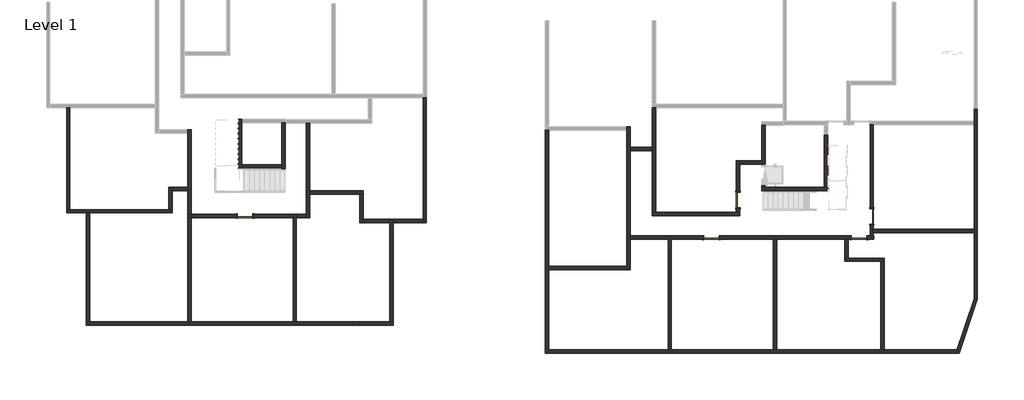
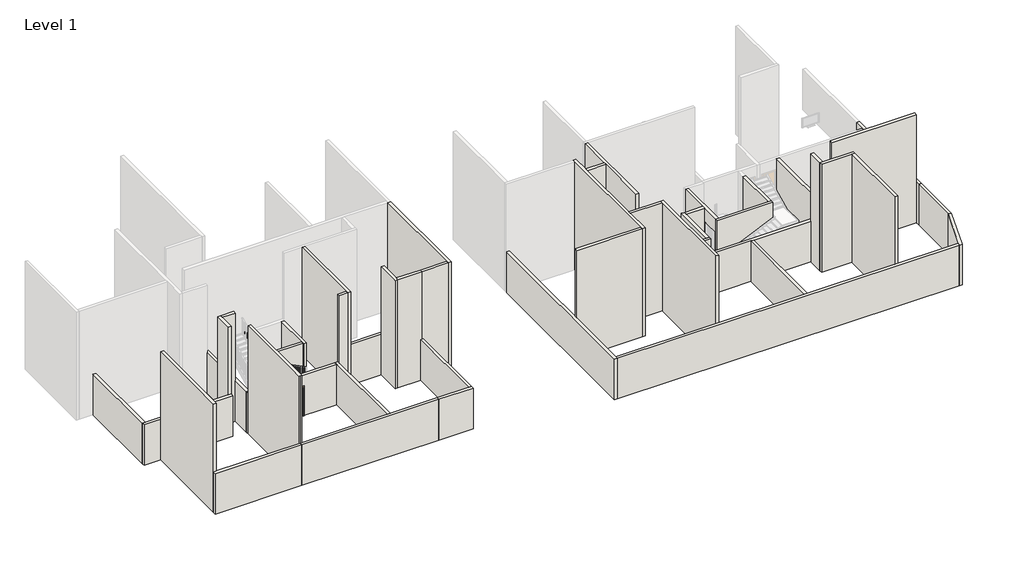
# One storey, part 1 of 3: 47 walls, 5 doors.
"""IFC4 building model written with IfcOpenShell, lengths in millimetres."""

import ifcopenshell
import ifcopenshell.guid

model = None  # the IFC model being written
_history = None  # IfcOwnerHistory: only IFC2X3 demands one
_inside = {}  # id of a spatial element -> (the spatial element, [elements in it])
_under = {}  # id of a project, library or spatial element -> (it, [spatial elements below it])
_declared = {}  # id of a project -> (the project, [libraries it declares])
_typed = {}  # id of a type object -> (the type object, [elements of that type])
_made_of = {}  # id of a material, layer set ... -> (it, [elements and type objects made of it])


def new_model(schema):
    """Start an empty IFC model of exactly this schema.

    Asked for "IFC4X3", IfcOpenShell would pick the latest addendum, in which some entities
    have other attributes; the version numbers below select the first issue.
    IFC2X3 requires an IfcOwnerHistory on every rooted entity: one is made here for all.
    """
    global model, _history
    if schema == "IFC4X3":
        model = ifcopenshell.file(schema_version=(4, 3, 0, 0))
    else:
        model = ifcopenshell.file(schema=schema)
    _inside.clear()
    _under.clear()
    _declared.clear()
    _typed.clear()
    _made_of.clear()
    _history = None
    if model.schema == "IFC2X3":
        org = make("IfcOrganization", Name="unknown")
        user = make(
            "IfcPersonAndOrganization",
            ThePerson=make("IfcPerson", FamilyName="unknown"),
            TheOrganization=org,
        )
        app = make(
            "IfcApplication",
            ApplicationDeveloper=org,
            Version="unknown",
            ApplicationFullName="unknown",
            ApplicationIdentifier="unknown",
        )
        _history = make(
            "IfcOwnerHistory",
            OwningUser=user,
            OwningApplication=app,
            ChangeAction="ADDED",
            CreationDate=0,
        )
    return model


def make(cls, **values):
    """One entity of the class cls with the attributes given. An attribute that is None is left unset."""
    return model.create_entity(
        cls, **{name: value for name, value in values.items() if value is not None}
    )


def rooted(cls, **values):
    """An entity with a GlobalId (a new one), such as an element, a storey or a relation."""
    return make(cls, GlobalId=ifcopenshell.guid.new(), OwnerHistory=_history, **values)


def si_unit(unit_type, name, prefix=None):
    """IfcSIUnit, for example si_unit("LENGTHUNIT", "METRE", prefix="MILLI")."""
    return make("IfcSIUnit", UnitType=unit_type, Prefix=prefix, Name=name)


def assignment(units):
    """IfcUnitAssignment: the units of a project."""
    return None if units is None else make("IfcUnitAssignment", Units=units)


def point(xyz):
    """IfcCartesianPoint."""
    return None if xyz is None else make("IfcCartesianPoint", Coordinates=xyz)


def direction(xyz):
    """IfcDirection."""
    return None if xyz is None else make("IfcDirection", DirectionRatios=xyz)


def frame(location, z_axis=None, x_axis=None):
    """IfcAxis2Placement3D, a coordinate frame: its origin and axes. An axis left out is left unset."""
    return make(
        "IfcAxis2Placement3D",
        Location=point(location),
        Axis=direction(z_axis),
        RefDirection=direction(x_axis),
    )


def origin():
    """The frame at (0, 0, 0) with its axes left unset."""
    return frame((0.0, 0.0, 0.0))


def origin_with_axes():
    """The frame at (0, 0, 0) with the z axis (0, 0, 1) and the x axis (1, 0, 0) written out."""
    return frame((0.0, 0.0, 0.0), z_axis=(0.0, 0.0, 1.0), x_axis=(1.0, 0.0, 0.0))


def place(relative_to, where):
    """IfcLocalPlacement: puts the frame where relative to a parent placement (None: the world)."""
    return make(
        "IfcLocalPlacement", PlacementRelTo=relative_to, RelativePlacement=where
    )


def context(
    kind, dimensions, precision=None, world=None, true_north=None, identifier=None
):
    """IfcGeometricRepresentationContext, for example the 3D "Model" context."""
    return make(
        "IfcGeometricRepresentationContext",
        ContextIdentifier=identifier,
        ContextType=kind,
        CoordinateSpaceDimension=dimensions,
        Precision=precision,
        WorldCoordinateSystem=world,
        TrueNorth=true_north,
    )


def project(units=None, contexts=None):
    """IfcProject with its units and contexts."""
    return rooted(
        "IfcProject",
        Name="project",
        RepresentationContexts=contexts,
        UnitsInContext=assignment(units),
    )


def spatial(cls, under=None, at=None, **own):
    """A site, building, storey or space (cls), placed at a placement, below another one or the project."""
    s = rooted(cls, ObjectPlacement=at, **own)
    if under is not None:
        _under.setdefault(under.id(), (under, []))[1].append(s)
    return s


def polyline(points):
    """IfcPolyline through the points."""
    return make("IfcPolyline", Points=[point(p) for p in points])


def outline(outer, holes=None, kind="AREA"):
    """IfcArbitraryClosedProfileDef: a profile drawn as a closed curve; with holes, ...WithVoids."""
    if holes is None:
        return make("IfcArbitraryClosedProfileDef", ProfileType=kind, OuterCurve=outer)
    return make(
        "IfcArbitraryProfileDefWithVoids",
        ProfileType=kind,
        OuterCurve=outer,
        InnerCurves=holes,
    )


def extrude(swept, where, along, depth):
    """IfcExtrudedAreaSolid: the profile swept, set in the frame where, extruded along a direction by depth."""
    return make(
        "IfcExtrudedAreaSolid",
        SweptArea=swept,
        Position=where,
        ExtrudedDirection=direction(along),
        Depth=depth,
    )


def faces_of(points, faces, orient=None, outer=None):
    """IfcFace entities. A face is a list of loops; a loop is a list of indices into points, from 0.

    orient and outer hold one flag for each loop. By default every Orientation is true, the
    first loop of a face is its IfcFaceOuterBound and the others are IfcFaceBound.
    """
    made = []
    for i, loops in enumerate(faces):
        bounds = []
        for j, loop in enumerate(loops):
            is_outer = j == 0 if outer is None else outer[i][j]
            bounds.append(
                make(
                    "IfcFaceOuterBound" if is_outer else "IfcFaceBound",
                    Bound=make("IfcPolyLoop", Polygon=[points[k] for k in loop]),
                    Orientation=True if orient is None else orient[i][j],
                )
            )
        made.append(make("IfcFace", Bounds=bounds))
    return made


def faceted_brep(points, faces, orient=None, outer=None, voids=None):
    """IfcFacetedBrep: a solid bounded by flat faces; with voids (closed shells), ...WithVoids."""
    shared = [point(p) for p in points]
    hull = make("IfcClosedShell", CfsFaces=faces_of(shared, faces, orient, outer))
    if voids is None:
        return make("IfcFacetedBrep", Outer=hull)
    return make(
        "IfcFacetedBrepWithVoids",
        Outer=hull,
        Voids=[
            make(cls, CfsFaces=faces_of(shared, fs, o, b)) for cls, fs, o, b in voids
        ],
    )


def shape(context_of_items, identifier, shape_type, items):
    """IfcShapeRepresentation: the items that make up one representation, for example the "Body"."""
    return make(
        "IfcShapeRepresentation",
        ContextOfItems=context_of_items,
        RepresentationIdentifier=identifier,
        RepresentationType=shape_type,
        Items=items,
    )


def source(mapping_origin, context_of_items, identifier, shape_type, items):
    """IfcRepresentationMap: a shape defined once, which mapped items show again and again."""
    return make(
        "IfcRepresentationMap",
        MappingOrigin=mapping_origin,
        MappedRepresentation=shape(context_of_items, identifier, shape_type, items),
    )


def transform(
    local_origin,
    x_axis=None,
    y_axis=None,
    z_axis=None,
    scale=None,
    scale2=None,
    scale3=None,
    uniform=True,
):
    """IfcCartesianTransformationOperator3D, or its non-uniform kind. x_axis, y_axis, z_axis: its Axis1, 2, 3."""
    if uniform:
        return make(
            "IfcCartesianTransformationOperator3D",
            Axis1=direction(x_axis),
            Axis2=direction(y_axis),
            LocalOrigin=point(local_origin),
            Scale=scale,
            Axis3=direction(z_axis),
        )
    return make(
        "IfcCartesianTransformationOperator3DnonUniform",
        Axis1=direction(x_axis),
        Axis2=direction(y_axis),
        LocalOrigin=point(local_origin),
        Scale=scale,
        Axis3=direction(z_axis),
        Scale2=scale2,
        Scale3=scale3,
    )


def mapped(mapping_source, mapping_target):
    """IfcMappedItem: shows the shape of a source again, moved by a transform."""
    return make(
        "IfcMappedItem", MappingSource=mapping_source, MappingTarget=mapping_target
    )


def made_of(thing, what):
    """Note that an element or type object is made of a material, layer set ...; save() writes the relation."""
    if what is not None:
        _made_of.setdefault(what.id(), (what, []))[1].append(thing)
    return thing


def element(
    cls,
    number,
    at=None,
    inside=None,
    cuts=None,
    type_object=None,
    material=None,
    context=None,
    identifier="Body",
    shape_type=None,
    held_by="IfcProductDefinitionShape",
    body=None,
    shapes=None,
    **own,
):
    """One element of the class cls, such as IfcWall. Its Tag is "e" and its number.

    at: its placement. inside: the storey or other place that contains it. cuts: it is an
    opening in that element (IfcRelVoidsElement). A single representation is given by context,
    identifier, shape_type and body (its items); several are given by shapes. held_by: the class
    of the entity that holds the representations. save() writes the other relations.
    """
    e = rooted(cls, Tag="e%d" % number, ObjectPlacement=at, **own)
    if body is not None:
        shapes = [shape(context, identifier, shape_type, body)]
    if shapes is not None:
        e.Representation = make(held_by, Representations=shapes)
    if inside is not None:
        _inside.setdefault(inside.id(), (inside, []))[1].append(e)
    if cuts is not None:
        rooted(
            "IfcRelVoidsElement", RelatingBuildingElement=cuts, RelatedOpeningElement=e
        )
    if type_object is not None:
        _typed.setdefault(type_object.id(), (type_object, []))[1].append(e)
    return made_of(e, material)


def aggregate(whole, parts):
    """IfcRelAggregates: a whole, such as a stair, and the parts it consists of."""
    return rooted("IfcRelAggregates", RelatingObject=whole, RelatedObjects=parts)


def save(model, path):
    """Write the relations noted so far, then the file.

    IfcRelAggregates (storeys below a building ...), IfcRelContainedInSpatialStructure (elements
    in a storey), IfcRelDefinesByType, IfcRelAssociatesMaterial and IfcRelDeclares: one each for
    every whole, place, type object, material and project.
    """
    for whole, parts in _under.values():
        aggregate(whole, parts)
    for where, things in _inside.values():
        rooted(
            "IfcRelContainedInSpatialStructure",
            RelatedElements=things,
            RelatingStructure=where,
        )
    for kind, things in _typed.values():
        rooted("IfcRelDefinesByType", RelatedObjects=things, RelatingType=kind)
    for what, things in _made_of.values():
        rooted("IfcRelAssociatesMaterial", RelatedObjects=things, RelatingMaterial=what)
    for by, libraries in _declared.values():
        rooted("IfcRelDeclares", RelatingContext=by, RelatedDefinitions=libraries)
    model.write(path)


def m_single_flush_0915_x_2134mm_727434cd(model_context):
    return source(origin(), model_context, "Body", "SweptSolid", [
        extrude(outline(polyline([(2210.0, -533.5), (0.0, -533.5), (0.0, -457.5), (2134.0, -457.5), (2134.0, 457.5), (0.0, 457.5), (0.0, 533.5), (2210.0, 533.5), (2210.0, -533.5)])), frame((0.0, -125.0, 0.0), z_axis=(0.0, 1.0, 0.0), x_axis=(0.0, 0.0, 1.0)), (0.0, 0.0, 1.0), 25.0),
        extrude(outline(polyline([(2210.0, 533.5), (2210.0, -533.5), (0.0, -533.5), (0.0, -457.5), (2134.0, -457.5), (2134.0, 457.5), (0.0, 457.5), (0.0, 533.5), (2210.0, 533.5)])), frame((0.0, 100.0, 0.0), z_axis=(0.0, 1.0, 0.0), x_axis=(0.0, 0.0, 1.0)), (0.0, 0.0, 1.0), 25.0),
        extrude(outline(polyline([(457.5, -49.0), (457.5, -100.0), (-457.5, -100.0), (-457.5, -49.0), (457.5, -49.0)])), origin_with_axes(), (0.0, 0.0, 1.0), 2134.0),
    ])


def m_single_flush_0915_x_2134mm_6a9e8738(model_context):
    return source(origin(), model_context, "Body", "SweptSolid", [
        extrude(outline(polyline([(2210.0, -533.5), (0.0, -533.5), (0.0, -457.5), (2134.0, -457.5), (2134.0, 457.5), (0.0, 457.5), (0.0, 533.5), (2210.0, 533.5), (2210.0, -533.5)])), frame((0.0, 100.0, 0.0), z_axis=(0.0, 1.0, 0.0), x_axis=(0.0, 0.0, 1.0)), (0.0, 0.0, 1.0), 25.0),
        extrude(outline(polyline([(2210.0, 533.5), (2210.0, -533.5), (0.0, -533.5), (0.0, -457.5), (2134.0, -457.5), (2134.0, 457.5), (0.0, 457.5), (0.0, 533.5), (2210.0, 533.5)])), frame((0.0, -125.0, 0.0), z_axis=(0.0, 1.0, 0.0), x_axis=(0.0, 0.0, 1.0)), (0.0, 0.0, 1.0), 25.0),
        extrude(outline(polyline([(457.5, 49.0), (-457.5, 49.0), (-457.5, 100.0), (457.5, 100.0), (457.5, 49.0)])), origin_with_axes(), (0.0, 0.0, 1.0), 2134.0),
    ])


model = new_model("IFC4")

# Units and contexts
model_context = context("Model", 3, world=origin())
ifc_project = project(units=[si_unit("LENGTHUNIT", "METRE", prefix="MILLI")], contexts=[model_context])

# Site, building, storey
site = spatial("IfcSite", under=ifc_project)
building = spatial("IfcBuilding", under=site)
storey = spatial("IfcBuildingStorey", under=building, Name="Level 1", Elevation=0.0)

# Doors
placement = place(None, origin())
m_single_flush_0915_x_2134mm_shape = m_single_flush_0915_x_2134mm_727434cd(model_context)
element("IfcDoor", 1, ObjectType="M_Single-Flush : 0915 x 2134mm", at=placement, inside=storey, context=model_context, shape_type="MappedRepresentation", body=[
    mapped(m_single_flush_0915_x_2134mm_shape, transform((16170.6041014, -4023.024372, 0.0), x_axis=(0.0, -1.0, 0.0), y_axis=(1.0, 0.0, 0.0), z_axis=(0.0, 0.0, 1.0))),
])
m_single_flush_0915_x_2134mm_2_shape = m_single_flush_0915_x_2134mm_6a9e8738(model_context)
element("IfcDoor", 2, ObjectType="M_Single-Flush : 0915 x 2134mm", at=placement, inside=storey, context=model_context, shape_type="MappedRepresentation", body=[
    mapped(m_single_flush_0915_x_2134mm_2_shape, transform((14602.336337, -6240.0098119, 0.0), x_axis=(-1.0, 0.0, 0.0), y_axis=(0.0, -1.0, 0.0), z_axis=(0.0, 0.0, 1.0))),
])
element("IfcDoor", 3, ObjectType="M_Single-Flush : 0915 x 2134mm", at=placement, inside=storey, context=model_context, shape_type="MappedRepresentation", body=[
    mapped(m_single_flush_0915_x_2134mm_2_shape, transform((24048.8612349, -4982.5098119, 0.0), x_axis=(0.0, -1.0, 0.0), y_axis=(1.0, 0.0, 0.0), z_axis=(0.0, 0.0, 1.0))),
])
element("IfcDoor", 4, ObjectType="M_Single-Flush : 0915 x 2134mm", at=placement, inside=storey, context=model_context, shape_type="MappedRepresentation", body=[
    mapped(m_single_flush_0915_x_2134mm_2_shape, transform((23308.8612349, -6240.0098119, 0.0), x_axis=(-1.0, 0.0, 0.0), y_axis=(0.0, -1.0, 0.0), z_axis=(0.0, 0.0, 1.0))),
])
element("IfcDoor", 5, ObjectType="M_Single-Flush : 0915 x 2134mm", at=placement, inside=storey, context=model_context, shape_type="MappedRepresentation", body=[
    mapped(m_single_flush_0915_x_2134mm_2_shape, transform((-12832.3304233, -4959.1627129, 0.0), x_axis=(-1.0, 0.0, 0.0), y_axis=(0.0, -1.0, 0.0), z_axis=(0.0, 0.0, 1.0))),
])

# Walls
element("IfcWall", 6, ObjectType="Generic - 200mm", at=placement, inside=storey, context=model_context, shape_type="Brep", body=[
    faceted_brep([(30068.8612349, 1319.475628, 0.0), (30068.8612349, 619.475628, 0.0), (30068.8612349, 419.475628, 0.0), (30068.8612349, -5760.0098119, 0.0), (30068.8612349, -5960.0098119, 0.0), (30068.8612349, -6240.0098119, 0.0), (30068.8612349, -6240.0098119, 3000.0), (30068.8612349, 419.475628, 3000.0), (30068.8612349, 619.475628, 3000.0), (30068.8612349, 1319.475628, 3000.0), (30268.8612349, 1319.475628, 0.0), (30268.8612349, 1319.475628, 3000.0), (30268.8612349, -6240.0098119, 3000.0), (30268.8612349, -6240.0098119, 0.0), (30268.3425199, 1319.475628, 0.0), (30069.3799498, -6240.0098119, 0.0), (30069.3799498, -6240.0098119, 3000.0), (30268.3425199, 1319.475628, 3000.0)], [[[0, 1, 2, 3, 4, 5, 6, 7, 8, 9]], [[10, 11, 12, 13]], [[5, 4, 3, 2, 1, 0, 14, 10, 13, 15]], [[6, 5, 15, 13, 12, 16]], [[9, 8, 7, 6, 16, 12, 11, 17]], [[0, 9, 17, 11, 10, 14]]]),
])
element("IfcWall", 7, ObjectType="Generic - 200mm", at=placement, inside=storey, context=model_context, shape_type="Brep", body=[
    faceted_brep([(30069.3799498, -6240.0098119, 0.0), (30069.3799498, -9831.8731192, 0.0), (30069.3799498, -9831.8731192, 3000.0), (30069.3799498, -6240.0098119, 3000.0), (30269.3799498, -6240.0098119, 0.0), (30269.3799498, -6240.0098119, 3000.0), (30269.3799498, -9864.7113693, 3000.0), (30269.3799498, -9864.7113693, 0.0), (30268.8612349, -6240.0098119, 0.0), (30268.8612349, -6240.0098119, 3000.0)], [[[0, 1, 2, 3]], [[4, 5, 6, 7]], [[1, 0, 8, 4, 7]], [[3, 2, 6, 5, 9]], [[0, 3, 9, 5, 4, 8]], [[2, 1, 7, 6]]]),
])
element("IfcWall", 8, ObjectType="Generic - 200mm", at=placement, inside=storey, context=model_context, shape_type="Brep", body=[
    faceted_brep([(21449.836337, -3276.2808257, 0.0), (21249.836337, -3276.2808257, 0.0), (17770.6041014, -3276.2808257, 0.0), (17570.6041014, -3276.2808257, 0.0), (17570.6041014, -3276.2808257, 3000.0), (17770.6041014, -3276.2808257, 3000.0), (21249.836337, -3276.2808257, 3000.0), (21449.836337, -3276.2808257, 3000.0), (21449.836337, -3476.2808257, 0.0), (21449.836337, -3476.2808257, 3000.0), (17570.6041014, -3476.2808257, 3000.0), (17570.6041014, -3476.2808257, 0.0)], [[[0, 1, 2, 3, 4, 5, 6, 7]], [[8, 9, 10, 11]], [[3, 2, 1, 0, 8, 11]], [[7, 6, 5, 4, 10, 9]], [[0, 7, 9, 8]], [[4, 3, 11, 10]]]),
])
element("IfcWall", 9, ObjectType="Generic - 200mm", at=placement, inside=storey, context=model_context, shape_type="SweptSolid", body=[
    extrude(outline(polyline([(18459.836337, -6340.0098119), (18459.836337, -12836.6907835), (18259.836337, -12836.6907835), (18259.836337, -6340.0098119), (18459.836337, -6340.0098119)])), origin_with_axes(), (0.0, 0.0, 1.0), 3000.0),
])
element("IfcWall", 10, ObjectType="Generic - 200mm", at=placement, inside=storey, context=model_context, shape_type="Brep", body=[
    faceted_brep([(29055.3124022, -12836.6907835, 0.0), (24788.8612349, -12836.6907835, 0.0), (24588.8612349, -12836.6907835, 0.0), (18459.836337, -12836.6907835, 0.0), (18259.836337, -12836.6907835, 0.0), (12259.836337, -12836.6907835, 0.0), (12059.836337, -12836.6907835, 0.0), (5043.716007, -12836.6907835, 0.0), (5043.716007, -12836.6907835, 3000.0), (18259.836337, -12836.6907835, 3000.0), (18459.836337, -12836.6907835, 3000.0), (29055.3124022, -12836.6907835, 3000.0), (28987.8162902, -13036.6907835, 0.0), (28987.8162902, -13036.6907835, 3000.0), (5043.716007, -13036.6907835, 3000.0), (5043.716007, -13036.6907835, 0.0)], [[[0, 1, 2, 3, 4, 5, 6, 7, 8, 9, 10, 11]], [[12, 13, 14, 15]], [[7, 6, 5, 4, 3, 2, 1, 0, 12, 15]], [[11, 10, 9, 8, 14, 13]], [[0, 11, 13, 12]], [[8, 7, 15, 14]]]),
])
element("IfcWall", 11, ObjectType="Generic - 200mm", at=placement, inside=storey, context=model_context, shape_type="Brep", body=[
    faceted_brep([(30069.3799498, -9831.8731192, 0.0), (29055.3124022, -12836.6907835, 0.0), (28987.8162902, -13036.6907835, 0.0), (28987.8162902, -13036.6907835, 3000.0), (29055.3124022, -12836.6907835, 3000.0), (30069.3799498, -9831.8731192, 3000.0), (30269.3799498, -9864.7113693, 0.0), (30269.3799498, -9864.7113693, 3000.0), (29198.8985612, -13036.6907835, 3000.0), (29198.8985612, -13036.6907835, 0.0)], [[[0, 1, 2, 3, 4, 5]], [[6, 7, 8, 9]], [[2, 1, 0, 6, 9]], [[5, 4, 3, 8, 7]], [[0, 5, 7, 6]], [[3, 2, 9, 8]]]),
])
element("IfcWall", 12, ObjectType="Generic - 200mm", at=placement, inside=storey, context=model_context, shape_type="Brep", body=[
    faceted_brep([(22851.3612349, -6140.0098119, 2134.0), (22851.3612349, -6140.0098119, 0.0), (15059.836337, -6140.0098119, 0.0), (15059.836337, -6140.0098119, 2134.0), (14144.836337, -6140.0098119, 2134.0), (14144.836337, -6140.0098119, 0.0), (12259.836337, -6140.0098119, 0.0), (12259.836337, -6140.0098119, 3000.0), (23948.8612349, -6140.0098119, 3000.0), (24148.8612349, -6140.0098119, 3000.0), (24163.3998354, -6140.0098119, 3000.0), (24163.3998354, -6140.0098119, 0.0), (24148.8612349, -6140.0098119, 0.0), (23948.8612349, -6140.0098119, 0.0), (23766.3612349, -6140.0098119, 0.0), (23766.3612349, -6140.0098119, 2134.0), (15059.836337, -6340.0098119, 0.0), (18259.836337, -6340.0098119, 0.0), (18459.836337, -6340.0098119, 0.0), (22468.8612349, -6340.0098119, 0.0), (22668.8612349, -6340.0098119, 0.0), (22851.3612349, -6340.0098119, 0.0), (22851.3612349, -6340.0098119, 2134.0), (23766.3612349, -6340.0098119, 2134.0), (23766.3612349, -6340.0098119, 0.0), (24163.3998354, -6340.0098119, 0.0), (24163.3998354, -6340.0098119, 3000.0), (18459.836337, -6340.0098119, 3000.0), (18259.836337, -6340.0098119, 3000.0), (12259.836337, -6340.0098119, 3000.0), (12259.836337, -6340.0098119, 0.0), (14144.836337, -6340.0098119, 0.0), (14144.836337, -6340.0098119, 2134.0), (15059.836337, -6340.0098119, 2134.0)], [[[0, 1, 2, 3, 4, 5, 6, 7, 8, 9, 10, 11, 12, 13, 14, 15]], [[16, 17, 18, 19, 20, 21, 22, 23, 24, 25, 26, 27, 28, 29, 30, 31, 32, 33]], [[30, 6, 5, 31]], [[2, 1, 21, 20, 19, 18, 17, 16]], [[14, 13, 12, 11, 25, 24]], [[10, 9, 8, 7, 29, 28, 27, 26]], [[11, 10, 26, 25]], [[4, 32, 31, 5]], [[33, 3, 2, 16]], [[3, 33, 32, 4]], [[22, 21, 1, 0]], [[23, 22, 0, 15]], [[24, 23, 15, 14]], [[7, 6, 30, 29]]]),
])
element("IfcWall", 13, ObjectType="Generic - 200mm", at=placement, inside=storey, context=model_context, shape_type="Brep", body=[
    faceted_brep([(4843.716007, 79.9901881, 0.0), (4843.716007, -13036.6907835, 0.0), (4843.716007, -13036.6907835, 3000.0), (4843.716007, 79.9901881, 3000.0), (5043.716007, 79.9901881, 0.0), (5043.716007, 79.9901881, 3000.0), (5043.716007, -12836.6907835, 3000.0), (5043.716007, -13036.6907835, 3000.0), (5043.716007, -13036.6907835, 0.0), (5043.716007, -12836.6907835, 0.0), (5043.716007, -8120.0098119, 0.0), (5043.716007, -7920.0098119, 0.0)], [[[0, 1, 2, 3]], [[4, 5, 6, 7, 8, 9, 10, 11]], [[1, 0, 4, 11, 10, 9, 8]], [[3, 2, 7, 6, 5]], [[2, 1, 8, 7]], [[0, 3, 5, 4]]]),
])
element("IfcWall", 14, ObjectType="Generic - 200mm", at=placement, inside=storey, context=model_context, shape_type="Brep", body=[
    faceted_brep([(24148.8612349, 419.475628, 3000.0), (24148.8612349, -6140.0098119, 3000.0), (24148.8612349, -6140.0098119, 0.0), (24148.8612349, -5960.0098119, 0.0), (24148.8612349, -5760.0098119, 0.0), (24148.8612349, -5440.0098119, 0.0), (24148.8612349, -5440.0098119, 2134.0), (24148.8612349, -4525.0098119, 2134.0), (24148.8612349, -4525.0098119, 0.0), (24148.8612349, 419.475628, 0.0), (23948.8612349, -6140.0098119, 3000.0), (23948.8612349, 419.475628, 3000.0), (23948.8612349, 419.475628, 0.0), (23948.8612349, -4525.0098119, 0.0), (23948.8612349, -4525.0098119, 2134.0), (23948.8612349, -5440.0098119, 2134.0), (23948.8612349, -5440.0098119, 0.0), (23948.8612349, -6140.0098119, 0.0)], [[[0, 1, 2, 3, 4, 5, 6, 7, 8, 9]], [[10, 11, 12, 13, 14, 15, 16, 17]], [[12, 9, 8, 13]], [[2, 17, 16, 5, 4, 3]], [[1, 0, 11, 10]], [[0, 9, 12, 11]], [[15, 6, 5, 16]], [[7, 14, 13, 8]], [[14, 7, 6, 15]], [[2, 1, 10, 17]]]),
])
element("IfcWall", 15, ObjectType="Generic - 200mm", at=placement, inside=storey, context=model_context, shape_type="SweptSolid", body=[
    extrude(outline(polyline([(21249.836337, -3276.2808257), (21249.836337, -200.524372), (21449.836337, -200.524372), (21449.836337, -3276.2808257), (21249.836337, -3276.2808257)])), origin_with_axes(), (0.0, 0.0, 1.0), 3000.0),
])
element("IfcWall", 16, ObjectType="Generic - 200mm", at=placement, inside=storey, context=model_context, shape_type="Brep", body=[
    faceted_brep([(17570.6041014, -3276.2808257, 3000.0), (17570.6041014, -1920.524372, 3000.0), (17570.6041014, -1720.524372, 3000.0), (17570.6041014, 379.475628, 3000.0), (17570.6041014, 379.475628, 0.0), (17570.6041014, -1720.524372, 0.0), (17570.6041014, -1920.524372, 0.0), (17570.6041014, -1926.2808257, 0.0), (17570.6041014, -1926.2808257, 2000.0), (17570.6041014, -3181.2876228, 2000.0), (17570.6041014, -3181.2876228, 0.0), (17570.6041014, -3276.2808257, 0.0), (17770.6041014, 379.475628, 3000.0), (17770.6041014, -3276.2808257, 3000.0), (17770.6041014, -3276.2808257, 0.0), (17770.6041014, -3181.2876228, 0.0), (17770.6041014, -3181.2876228, 2000.0), (17770.6041014, -1926.2808257, 2000.0), (17770.6041014, -1926.2808257, 0.0), (17770.6041014, 379.475628, 0.0)], [[[0, 1, 2, 3, 4, 5, 6, 7, 8, 9, 10, 11]], [[12, 13, 14, 15, 16, 17, 18, 19]], [[14, 11, 10, 15]], [[4, 19, 18, 7, 6, 5]], [[3, 2, 1, 0, 13, 12]], [[0, 11, 14, 13]], [[9, 16, 15, 10]], [[17, 8, 7, 18]], [[8, 17, 16, 9]], [[4, 3, 12, 19]]]),
])
element("IfcWall", 17, ObjectType="Generic - 200mm", at=placement, inside=storey, context=model_context, shape_type="Brep", body=[
    faceted_brep([(11128.8612349, -4940.0098119, 0.0), (16270.6041014, -4940.0098119, 0.0), (16270.6041014, -4940.0098119, 3000.0), (11128.8612349, -4940.0098119, 3000.0), (11128.8612349, -4740.0098119, 0.0), (11128.8612349, -4740.0098119, 3000.0), (16070.6041014, -4740.0098119, 3000.0), (16270.6041014, -4740.0098119, 3000.0), (16270.6041014, -4740.0098119, 0.0), (16070.6041014, -4740.0098119, 0.0), (11328.8612349, -4740.0098119, 0.0)], [[[0, 1, 2, 3]], [[4, 5, 6, 7, 8, 9, 10]], [[1, 0, 4, 10, 9, 8]], [[3, 2, 7, 6, 5]], [[2, 1, 8, 7]], [[0, 3, 5, 4]]]),
])
element("IfcWall", 18, ObjectType="Generic - 200mm", at=placement, inside=storey, context=model_context, shape_type="Brep", body=[
    faceted_brep([(16270.6041014, -1720.524372, 3000.0), (16270.6041014, -1920.524372, 3000.0), (16270.6041014, -4740.0098119, 3000.0), (16270.6041014, -4740.0098119, 0.0), (16270.6041014, -4480.524372, 0.0), (16270.6041014, -4480.524372, 2134.0), (16270.6041014, -3565.524372, 2134.0), (16270.6041014, -3565.524372, 0.0), (16270.6041014, -1920.524372, 0.0), (16270.6041014, -1720.524372, 0.0), (16070.6041014, -4740.0098119, 3000.0), (16070.6041014, -1720.524372, 3000.0), (16070.6041014, -1720.524372, 0.0), (16070.6041014, -3565.524372, 0.0), (16070.6041014, -3565.524372, 2134.0), (16070.6041014, -4480.524372, 2134.0), (16070.6041014, -4480.524372, 0.0), (16070.6041014, -4740.0098119, 0.0)], [[[0, 1, 2, 3, 4, 5, 6, 7, 8, 9]], [[10, 11, 12, 13, 14, 15, 16, 17]], [[3, 17, 16, 4]], [[12, 9, 8, 7, 13]], [[2, 1, 0, 11, 10]], [[3, 2, 10, 17]], [[0, 9, 12, 11]], [[15, 5, 4, 16]], [[6, 14, 13, 7]], [[14, 6, 5, 15]]]),
])
element("IfcWall", 19, ObjectType="Generic - 200mm", at=placement, inside=storey, context=model_context, shape_type="SweptSolid", body=[
    extrude(outline(polyline([(17570.6041014, -1920.524372), (16270.6041014, -1920.524372), (16270.6041014, -1720.524372), (17570.6041014, -1720.524372), (17570.6041014, -1920.524372)])), origin_with_axes(), (0.0, 0.0, 1.0), 3000.0),
])
element("IfcWall", 20, ObjectType="Generic - 200mm", at=placement, inside=storey, context=model_context, shape_type="Brep", body=[
    faceted_brep([(22468.8612349, -7641.2808257, 0.0), (24588.8612349, -7641.2808257, 0.0), (24788.8612349, -7641.2808257, 0.0), (24788.8612349, -7641.2808257, 8000.0), (24588.8612349, -7641.2808257, 8000.0), (22468.8612349, -7641.2808257, 8000.0), (22468.8612349, -7441.2808257, 0.0), (22468.8612349, -7441.2808257, 8000.0), (22668.8612349, -7441.2808257, 8000.0), (24788.8612349, -7441.2808257, 8000.0), (24788.8612349, -7441.2808257, 0.0), (22668.8612349, -7441.2808257, 0.0)], [[[0, 1, 2, 3, 4, 5]], [[6, 7, 8, 9, 10, 11]], [[2, 1, 0, 6, 11, 10]], [[5, 4, 3, 9, 8, 7]], [[3, 2, 10, 9]], [[0, 5, 7, 6]]]),
])
element("IfcWall", 21, ObjectType="Generic - 200mm", at=placement, inside=storey, context=model_context, shape_type="SweptSolid", body=[
    extrude(outline(polyline([(24588.8612349, -12836.6907835), (24588.8612349, -7641.2808257), (24788.8612349, -7641.2808257), (24788.8612349, -12836.6907835), (24588.8612349, -12836.6907835)])), origin_with_axes(), (0.0, 0.0, 1.0), 8000.0),
])
element("IfcWall", 22, ObjectType="Generic - 200mm", at=placement, inside=storey, context=model_context, shape_type="SweptSolid", body=[
    extrude(outline(polyline([(22668.8612349, -6340.0098119), (22668.8612349, -7441.2808257), (22468.8612349, -7441.2808257), (22468.8612349, -6340.0098119), (22668.8612349, -6340.0098119)])), origin_with_axes(), (0.0, 0.0, 1.0), 8000.0),
])
element("IfcWall", 23, ObjectType="Generic - 200mm", at=placement, inside=storey, context=model_context, shape_type="SweptSolid", body=[
    extrude(outline(polyline([(30068.8612349, -5960.0098119), (24148.8612349, -5960.0098119), (24148.8612349, -5760.0098119), (30068.8612349, -5760.0098119), (30068.8612349, -5960.0098119)])), origin_with_axes(), (0.0, 0.0, 1.0), 8000.0),
])
element("IfcWall", 24, ObjectType="Generic - 200mm", at=placement, inside=storey, context=model_context, shape_type="Brep", body=[
    faceted_brep([(9628.8612349, 279.9901881, 0.0), (9628.8612349, 79.9901881, 0.0), (9628.8612349, -7920.0098119, 0.0), (9628.8612349, -8120.0098119, 0.0), (9628.8612349, -8120.0098119, 8000.0), (9628.8612349, -7920.0098119, 8000.0), (9628.8612349, 79.9901881, 8000.0), (9628.8612349, 279.9901881, 8000.0), (9828.8612349, 279.9901881, 0.0), (9828.8612349, 279.9901881, 8000.0), (9828.8612349, -920.524372, 8000.0), (9828.8612349, -1120.524372, 8000.0), (9828.8612349, -6136.6907835, 8000.0), (9828.8612349, -6336.6907835, 8000.0), (9828.8612349, -8120.0098119, 8000.0), (9828.8612349, -8120.0098119, 0.0), (9828.8612349, -6336.6907835, 0.0), (9828.8612349, -6136.6907835, 0.0), (9828.8612349, -1120.524372, 0.0), (9828.8612349, -920.524372, 0.0)], [[[0, 1, 2, 3, 4, 5, 6, 7]], [[8, 9, 10, 11, 12, 13, 14, 15, 16, 17, 18, 19]], [[3, 2, 1, 0, 8, 19, 18, 17, 16, 15]], [[7, 6, 5, 4, 14, 13, 12, 11, 10, 9]], [[0, 7, 9, 8]], [[4, 3, 15, 14]]]),
])
element("IfcWall", 25, ObjectType="Generic - 200mm", at=placement, inside=storey, context=model_context, shape_type="SweptSolid", body=[
    extrude(outline(polyline([(5043.716007, -7920.0098119), (9628.8612349, -7920.0098119), (9628.8612349, -8120.0098119), (5043.716007, -8120.0098119), (5043.716007, -7920.0098119)])), origin_with_axes(), (0.0, 0.0, 1.0), 8000.0),
])
element("IfcWall", 26, ObjectType="Generic - 200mm", at=placement, inside=storey, context=model_context, shape_type="Brep", body=[
    faceted_brep([(-4309.8304233, -5158.643998, 0.0), (-4309.8304233, -5358.643998, 0.0), (-4309.8304233, -11188.643998, 0.0), (-4309.8304233, -11188.643998, 3000.0), (-4309.8304233, -5358.643998, 3000.0), (-4309.8304233, -5158.643998, 3000.0), (-4109.8304233, -5158.643998, 0.0), (-4109.8304233, -5158.643998, 3000.0), (-4109.8304233, -5358.643998, 3000.0), (-4109.8304233, -11188.643998, 3000.0), (-4109.8304233, -11188.643998, 0.0), (-4109.8304233, -5358.643998, 0.0), (-4209.8304233, -5158.643998, 3000.0)], [[[0, 1, 2, 3, 4, 5]], [[6, 7, 8, 9, 10, 11]], [[2, 1, 0, 6, 11, 10]], [[5, 4, 3, 9, 8, 7, 12]], [[3, 2, 10, 9]], [[0, 5, 12, 7, 6]]]),
])
element("IfcWall", 27, ObjectType="Generic - 200mm", at=placement, inside=storey, context=model_context, shape_type="Brep", body=[
    faceted_brep([(-4109.8304233, -11188.643998, 0.0), (-4309.8304233, -11188.643998, 0.0), (-6530.3449834, -11188.643998, 0.0), (-6530.3449834, -11188.643998, 3000.0), (-4309.8304233, -11188.643998, 3000.0), (-4109.8304233, -11188.643998, 3000.0), (-4109.8304233, -11388.643998, 0.0), (-4109.8304233, -11388.643998, 3000.0), (-6530.3449834, -11388.643998, 3000.0), (-6530.3449834, -11388.643998, 0.0), (-6530.3449834, -11189.1627129, 0.0), (-6530.3449834, -11189.1627129, 3000.0)], [[[0, 1, 2, 3, 4, 5]], [[6, 7, 8, 9]], [[2, 1, 0, 6, 9, 10]], [[3, 2, 10, 9, 8, 11]], [[5, 4, 3, 11, 8, 7]], [[0, 5, 7, 6]]]),
])
element("IfcWall", 28, ObjectType="Generic - 200mm", at=placement, inside=storey, context=model_context, shape_type="Brep", body=[
    faceted_brep([(-6530.3449834, -11189.1627129, 0.0), (-9814.8304233, -11189.1627129, 0.0), (-10014.8304233, -11189.1627129, 0.0), (-16014.8304233, -11189.1627129, 0.0), (-16114.8304233, -11189.1627129, 0.0), (-16114.8304233, -11189.1627129, 3000.0), (-10014.8304233, -11189.1627129, 3000.0), (-9814.8304233, -11189.1627129, 3000.0), (-6530.3449834, -11189.1627129, 3000.0), (-6530.3449834, -11389.1627129, 0.0), (-6530.3449834, -11389.1627129, 3000.0), (-16114.8304233, -11389.1627129, 3000.0), (-16114.8304233, -11389.1627129, 0.0), (-6530.3449834, -11388.643998, 0.0), (-16114.8304233, -11189.6814279, 0.0), (-16114.8304233, -11189.6814279, 3000.0), (-6530.3449834, -11388.643998, 3000.0)], [[[0, 1, 2, 3, 4, 5, 6, 7, 8]], [[9, 10, 11, 12]], [[4, 3, 2, 1, 0, 13, 9, 12, 14]], [[5, 4, 14, 12, 11, 15]], [[8, 7, 6, 5, 15, 11, 10, 16]], [[0, 8, 16, 10, 9, 13]]]),
])
element("IfcWall", 29, ObjectType="Generic - 200mm", at=placement, inside=storey, context=model_context, shape_type="Brep", body=[
    faceted_brep([(-16114.8304233, -11189.6814279, 0.0), (-16214.8304233, -11189.6814279, 0.0), (-21985.6447259, -11189.6814279, 0.0), (-22185.6447259, -11189.6814279, 0.0), (-22185.6447259, -11189.6814279, 3000.0), (-16114.8304233, -11189.6814279, 3000.0), (-16114.8304233, -11389.6814279, 0.0), (-16114.8304233, -11389.6814279, 3000.0), (-22185.6447259, -11389.6814279, 3000.0), (-22185.6447259, -11389.6814279, 0.0), (-16114.8304233, -11389.1627129, 0.0), (-16114.8304233, -11389.1627129, 3000.0)], [[[0, 1, 2, 3, 4, 5]], [[6, 7, 8, 9]], [[3, 2, 1, 0, 10, 6, 9]], [[5, 4, 8, 7, 11]], [[0, 5, 11, 7, 6, 10]], [[4, 3, 9, 8]]]),
])
element("IfcWall", 30, ObjectType="Generic - 200mm", at=placement, inside=storey, context=model_context, shape_type="Brep", body=[
    faceted_brep([(-13026.101437, -2140.1378151, 0.0), (-13026.101437, -1940.1378151, 0.0), (-13026.101437, 520.8372871, 0.0), (-13026.101437, 720.8372871, 0.0), (-13026.101437, 720.8372871, 3000.0), (-13026.101437, 520.8372871, 3000.0), (-13026.101437, -1940.1378151, 3000.0), (-13026.101437, -2140.1378151, 3000.0), (-13226.101437, -2140.1378151, 0.0), (-13226.101437, -2140.1378151, 3000.0), (-13226.101437, 720.8372871, 3000.0), (-13226.101437, 720.8372871, 0.0)], [[[0, 1, 2, 3, 4, 5, 6, 7]], [[8, 9, 10, 11]], [[3, 2, 1, 0, 8, 11]], [[7, 6, 5, 4, 10, 9]], [[0, 7, 9, 8]], [[4, 3, 11, 10]]]),
])
element("IfcWall", 31, ObjectType="Generic - 200mm", at=placement, inside=storey, context=model_context, shape_type="Brep", body=[
    faceted_brep([(-23346.5113948, -4787.1599715, 0.0), (-22185.6447259, -4787.1599715, 0.0), (-21985.6447259, -4787.1599715, 0.0), (-17123.9741722, -4787.1599715, 0.0), (-17123.9741722, -4787.1599715, 3000.0), (-23346.5113948, -4787.1599715, 3000.0), (-23346.5113948, -4587.1599715, 0.0), (-23346.5113948, -4587.1599715, 3000.0), (-23146.5113948, -4587.1599715, 3000.0), (-17123.9741722, -4587.1599715, 3000.0), (-17123.9741722, -4587.1599715, 0.0), (-17323.9741722, -4587.1599715, 0.0), (-23146.5113948, -4587.1599715, 0.0)], [[[0, 1, 2, 3, 4, 5]], [[6, 7, 8, 9, 10, 11, 12]], [[3, 2, 1, 0, 6, 12, 11, 10]], [[4, 3, 10, 9]], [[5, 4, 9, 8, 7]], [[0, 5, 7, 6]]]),
])
element("IfcWall", 32, ObjectType="Generic - 200mm", at=placement, inside=storey, context=model_context, shape_type="SweptSolid", body=[
    extrude(outline(polyline([(-23146.5113948, 1412.8400285), (-23146.5113948, -4587.1599715), (-23346.5113948, -4587.1599715), (-23346.5113948, 1412.8400285), (-23146.5113948, 1412.8400285)])), origin_with_axes(), (0.0, 0.0, 1.0), 3000.0),
])
element("IfcWall", 33, ObjectType="Generic - 200mm", at=placement, inside=storey, context=model_context, shape_type="Brep", body=[
    faceted_brep([(-16013.9741722, -4859.1627129, 0.0), (-16013.9741722, 112.8400285, 0.0), (-16013.9741722, 112.8400285, 3000.0), (-16013.9741722, -4859.1627129, 3000.0), (-16213.9741722, -4859.1627129, 0.0), (-16213.9741722, -4859.1627129, 3000.0), (-16213.9741722, 112.8400285, 3000.0), (-16213.9741722, 112.8400285, 0.0), (-16213.9741722, -87.1599715, 0.0), (-16213.9741722, -3287.1599715, 0.0), (-16213.9741722, -3487.1599715, 0.0)], [[[0, 1, 2, 3]], [[4, 5, 6, 7, 8, 9, 10]], [[1, 0, 4, 10, 9, 8, 7]], [[3, 2, 6, 5]], [[2, 1, 7, 6]], [[0, 3, 5, 4]]]),
])
element("IfcWall", 34, ObjectType="Generic - 200mm", at=placement, inside=storey, context=model_context, shape_type="Brep", body=[
    faceted_brep([(-10014.8304233, -5059.1627129, 3000.0), (-16213.9741722, -5059.1627129, 3000.0), (-16213.9741722, -5059.1627129, 0.0), (-16014.8304233, -5059.1627129, 0.0), (-13289.8304233, -5059.1627129, 0.0), (-13289.8304233, -5059.1627129, 2134.0), (-12374.8304233, -5059.1627129, 2134.0), (-12374.8304233, -5059.1627129, 0.0), (-10014.8304233, -5059.1627129, 0.0), (-16213.9741722, -4859.1627129, 3000.0), (-16013.9741722, -4859.1627129, 3000.0), (-10014.8304233, -4859.1627129, 3000.0), (-10014.8304233, -4859.1627129, 0.0), (-12374.8304233, -4859.1627129, 0.0), (-12374.8304233, -4859.1627129, 2134.0), (-13289.8304233, -4859.1627129, 2134.0), (-13289.8304233, -4859.1627129, 0.0), (-16013.9741722, -4859.1627129, 0.0), (-16213.9741722, -4859.1627129, 0.0)], [[[0, 1, 2, 3, 4, 5, 6, 7, 8]], [[9, 10, 11, 12, 13, 14, 15, 16, 17, 18]], [[12, 8, 7, 13]], [[2, 18, 17, 16, 4, 3]], [[1, 0, 11, 10, 9]], [[0, 8, 12, 11]], [[15, 5, 4, 16]], [[6, 14, 13, 7]], [[14, 6, 5, 15]], [[2, 1, 9, 18]]]),
])
element("IfcWall", 35, ObjectType="Generic - 200mm", at=placement, inside=storey, context=model_context, shape_type="SweptSolid", body=[
    extrude(outline(polyline([(-13026.101437, -1940.1378151), (-10669.8304233, -1940.1378151), (-10669.8304233, -2140.1378151), (-13026.101437, -2140.1378151), (-13026.101437, -1940.1378151)])), origin_with_axes(), (0.0, 0.0, 1.0), 3000.0),
])
element("IfcWall", 36, ObjectType="Generic - 200mm", at=placement, inside=storey, context=model_context, shape_type="Brep", body=[
    faceted_brep([(-9030.3629108, -3680.1378151, 0.0), (-6095.3449834, -3680.1378151, 0.0), (-5895.3449834, -3680.1378151, 0.0), (-5895.3449834, -3680.1378151, 3000.0), (-9030.3629108, -3680.1378151, 3000.0), (-9030.3629108, -3480.1378151, 0.0), (-9030.3629108, -3480.1378151, 3000.0), (-5895.3449834, -3480.1378151, 3000.0), (-5895.3449834, -3480.1378151, 0.0)], [[[0, 1, 2, 3, 4]], [[5, 6, 7, 8]], [[2, 1, 0, 5, 8]], [[4, 3, 7, 6]], [[3, 2, 8, 7]], [[0, 4, 6, 5]]]),
])
element("IfcWall", 37, ObjectType="Generic - 200mm", at=placement, inside=storey, context=model_context, shape_type="Brep", body=[
    faceted_brep([(-10014.8304233, -4859.1627129, 0.0), (-10014.8304233, -5059.1627129, 0.0), (-10014.8304233, -11189.1627129, 0.0), (-10014.8304233, -11189.1627129, 3000.0), (-10014.8304233, -5059.1627129, 3000.0), (-10014.8304233, -4859.1627129, 3000.0), (-9814.8304233, -4859.1627129, 0.0), (-9814.8304233, -4859.1627129, 3000.0), (-9814.8304233, -11189.1627129, 3000.0), (-9814.8304233, -11189.1627129, 0.0), (-9814.8304233, -5059.1627129, 0.0)], [[[0, 1, 2, 3, 4, 5]], [[6, 7, 8, 9, 10]], [[2, 1, 0, 6, 10, 9]], [[5, 4, 3, 8, 7]], [[3, 2, 9, 8]], [[0, 5, 7, 6]]]),
])
element("IfcWall", 38, ObjectType="Generic - 200mm", at=placement, inside=storey, context=model_context, shape_type="Brep", body=[
    faceted_brep([(-10469.8304233, -2179.1627129, 0.0), (-10469.8304233, 500.8372871, 0.0), (-10469.8304233, 520.8372871, 0.0), (-10469.8304233, 520.8372871, 3000.0), (-10469.8304233, -2179.1627129, 3000.0), (-10669.8304233, -2179.1627129, 0.0), (-10669.8304233, -2179.1627129, 3000.0), (-10669.8304233, -2140.1378151, 3000.0), (-10669.8304233, -1940.1378151, 3000.0), (-10669.8304233, 520.8372871, 3000.0), (-10669.8304233, 520.8372871, 0.0), (-10669.8304233, -1940.1378151, 0.0), (-10669.8304233, -2140.1378151, 0.0)], [[[0, 1, 2, 3, 4]], [[5, 6, 7, 8, 9, 10, 11, 12]], [[2, 1, 0, 5, 12, 11, 10]], [[4, 3, 9, 8, 7, 6]], [[0, 4, 6, 5]], [[3, 2, 10, 9]]]),
])
element("IfcWall", 39, ObjectType="Generic - 200mm", at=placement, inside=storey, context=model_context, shape_type="Brep", body=[
    faceted_brep([(-6095.3449834, -3680.1378151, 0.0), (-6095.3449834, -5358.643998, 0.0), (-6095.3449834, -5358.643998, 8000.0), (-6095.3449834, -3680.1378151, 8000.0), (-5895.3449834, -3680.1378151, 0.0), (-5895.3449834, -3680.1378151, 3000.0), (-5895.3449834, -3680.1378151, 8000.0), (-5895.3449834, -5158.643998, 8000.0), (-5895.3449834, -5358.643998, 8000.0), (-5895.3449834, -5358.643998, 0.0), (-5895.3449834, -5158.643998, 0.0)], [[[0, 1, 2, 3]], [[4, 5, 6, 7, 8, 9, 10]], [[1, 0, 4, 10, 9]], [[3, 2, 8, 7, 6]], [[2, 1, 9, 8]], [[0, 3, 6, 5, 4]]]),
])
element("IfcWall", 40, ObjectType="Generic - 200mm", at=placement, inside=storey, context=model_context, shape_type="SweptSolid", body=[
    extrude(outline(polyline([(0.0, -5895.3449834), (0.0, -4309.8304233), (3000.0, -4309.8304233), (3000.0, -4209.8304233), (8000.0, -4209.8304233), (8000.0, -5895.3449834), (0.0, -5895.3449834)])), frame((0.0, -5358.643998, 0.0), z_axis=(0.0, 1.0, 0.0), x_axis=(0.0, 0.0, 1.0)), (0.0, 0.0, 1.0), 200.0),
])
element("IfcWall", 41, ObjectType="Generic - 200mm", at=placement, inside=storey, context=model_context, shape_type="Brep", body=[
    faceted_brep([(12059.836337, -6136.6907835, 0.0), (12059.836337, -6336.6907835, 0.0), (12059.836337, -12836.6907835, 0.0), (12059.836337, -12836.6907835, 8000.0), (12059.836337, -6336.6907835, 8000.0), (12059.836337, -6136.6907835, 8000.0), (12259.836337, -6136.6907835, 0.0), (12259.836337, -6136.6907835, 8000.0), (12259.836337, -12836.6907835, 8000.0), (12259.836337, -12836.6907835, 0.0), (12259.836337, -6340.0098119, 0.0), (12259.836337, -6140.0098119, 0.0)], [[[0, 1, 2, 3, 4, 5]], [[6, 7, 8, 9, 10, 11]], [[2, 1, 0, 6, 11, 10, 9]], [[5, 4, 3, 8, 7]], [[3, 2, 9, 8]], [[0, 5, 7, 6]]]),
])
element("IfcWall", 42, ObjectType="Generic - 200mm", at=placement, inside=storey, context=model_context, shape_type="SweptSolid", body=[
    extrude(outline(polyline([(12059.836337, -6336.6907835), (9828.8612349, -6336.6907835), (9828.8612349, -6136.6907835), (12059.836337, -6136.6907835), (12059.836337, -6336.6907835)])), origin_with_axes(), (0.0, 0.0, 1.0), 8000.0),
])
element("IfcWall", 43, ObjectType="Generic - 200mm", at=placement, inside=storey, context=model_context, shape_type="SweptSolid", body=[
    extrude(outline(polyline([(0.0, -4109.8304233), (0.0, -2360.3449834), (8000.0, -2360.3449834), (8000.0, -4209.8304233), (3000.0, -4209.8304233), (3000.0, -4109.8304233), (0.0, -4109.8304233)])), frame((0.0, -5358.643998, 0.0), z_axis=(0.0, 1.0, 0.0), x_axis=(0.0, 0.0, 1.0)), (0.0, 0.0, 1.0), 200.0),
])
element("IfcWall", 44, ObjectType="Generic - 200mm", at=placement, inside=storey, context=model_context, shape_type="Brep", body=[
    faceted_brep([(-16214.8304233, -5059.1627129, 0.0), (-16214.8304233, -11189.6814279, 0.0), (-16214.8304233, -11189.6814279, 8000.0), (-16214.8304233, -5059.1627129, 8000.0), (-16014.8304233, -5059.1627129, 0.0), (-16014.8304233, -5059.1627129, 8000.0), (-16014.8304233, -11189.1627129, 8000.0), (-16014.8304233, -11189.1627129, 0.0), (-16213.9741722, -5059.1627129, 0.0), (-16114.8304233, -11189.1627129, 0.0), (-16114.8304233, -11189.6814279, 0.0), (-16114.8304233, -11189.6814279, 8000.0), (-16114.8304233, -11189.1627129, 8000.0), (-16114.8304233, -11189.6814279, 3000.0), (-16114.8304233, -11189.1627129, 3000.0)], [[[0, 1, 2, 3]], [[4, 5, 6, 7]], [[1, 0, 8, 4, 7, 9, 10]], [[3, 2, 11, 12, 6, 5]], [[2, 1, 10, 13, 11]], [[10, 9, 14, 12, 11, 13]], [[9, 7, 6, 12, 14]], [[0, 3, 5, 4, 8]]]),
])
element("IfcWall", 45, ObjectType="Generic - 200mm", at=placement, inside=storey, context=model_context, shape_type="Brep", body=[
    faceted_brep([(-21985.6447259, -11189.6814279, 0.0), (-21985.6447259, -4787.1599715, 0.0), (-21985.6447259, -4787.1599715, 8000.0), (-21985.6447259, -11189.6814279, 8000.0), (-22185.6447259, -11189.6814279, 0.0), (-22185.6447259, -11189.6814279, 3000.0), (-22185.6447259, -11189.6814279, 8000.0), (-22185.6447259, -4787.1599715, 8000.0), (-22185.6447259, -4787.1599715, 0.0)], [[[0, 1, 2, 3]], [[4, 5, 6, 7, 8]], [[1, 0, 4, 8]], [[3, 2, 7, 6]], [[2, 1, 8, 7]], [[0, 3, 6, 5, 4]]]),
])
element("IfcWall", 46, ObjectType="Generic - 200mm", at=placement, inside=storey, context=model_context, shape_type="Brep", body=[
    faceted_brep([(-2360.3449834, 2000.8372871, 0.0), (-2360.3449834, -5158.643998, 0.0), (-2360.3449834, -5358.643998, 0.0), (-2360.3449834, -5358.643998, 8000.0), (-2360.3449834, -5158.643998, 8000.0), (-2360.3449834, 2000.8372871, 8000.0), (-2160.3449834, 2000.8372871, 0.0), (-2160.3449834, 2000.8372871, 8000.0), (-2160.3449834, -5358.643998, 8000.0), (-2160.3449834, -5358.643998, 0.0), (-2350.3449834, 2000.8372871, 0.0), (-2350.3449834, 2000.8372871, 8000.0)], [[[0, 1, 2, 3, 4, 5]], [[6, 7, 8, 9]], [[2, 1, 0, 10, 6, 9]], [[5, 4, 3, 8, 7, 11]], [[3, 2, 9, 8]], [[0, 5, 11, 7, 6, 10]]]),
])
element("IfcWall", 47, ObjectType="Generic - 200mm", at=placement, inside=storey, context=model_context, shape_type="Brep", body=[
    faceted_brep([(-9230.3629108, 500.8372871, 0.0), (-9230.3629108, -4859.1627129, 0.0), (-9230.3629108, -5059.1627129, 0.0), (-9230.3629108, -5059.1627129, 8000.0), (-9230.3629108, -4859.1627129, 8000.0), (-9230.3629108, 500.8372871, 8000.0), (-9030.3629108, 500.8372871, 0.0), (-9030.3629108, 500.8372871, 8000.0), (-9030.3629108, -5059.1627129, 8000.0), (-9030.3629108, -5059.1627129, 0.0), (-9030.3629108, -3680.1378151, 0.0), (-9030.3629108, -3480.1378151, 0.0)], [[[0, 1, 2, 3, 4, 5]], [[6, 7, 8, 9, 10, 11]], [[2, 1, 0, 6, 11, 10, 9]], [[5, 4, 3, 8, 7]], [[0, 5, 7, 6]], [[3, 2, 9, 8]]]),
])
element("IfcWall", 48, ObjectType="Generic - 200mm", at=placement, inside=storey, context=model_context, shape_type="Brep", body=[
    faceted_brep([(-9814.8304233, -5059.1627129, 0.0), (-9230.3629108, -5059.1627129, 0.0), (-9230.3629108, -5059.1627129, 8000.0), (-9814.8304233, -5059.1627129, 8000.0), (-9814.8304233, -4859.1627129, 0.0), (-9814.8304233, -4859.1627129, 3000.0), (-9814.8304233, -4859.1627129, 8000.0), (-9230.3629108, -4859.1627129, 8000.0), (-9230.3629108, -4859.1627129, 0.0)], [[[0, 1, 2, 3]], [[4, 5, 6, 7, 8]], [[1, 0, 4, 8]], [[3, 2, 7, 6]], [[0, 3, 6, 5, 4]], [[2, 1, 8, 7]]]),
])
element("IfcWall", 49, ObjectType="Generic - 200mm", at=placement, inside=storey, context=model_context, shape_type="Brep", body=[
    faceted_brep([(11328.8612349, -4740.0098119, 0.0), (11328.8612349, 1419.475628, 0.0), (11328.8612349, 1419.475628, 8000.0), (11328.8612349, -4740.0098119, 8000.0), (11128.8612349, -4740.0098119, 0.0), (11128.8612349, -4740.0098119, 3000.0), (11128.8612349, -4740.0098119, 8000.0), (11128.8612349, -1120.524372, 8000.0), (11128.8612349, -920.524372, 8000.0), (11128.8612349, 1419.475628, 8000.0), (11128.8612349, 1419.475628, 0.0), (11128.8612349, -920.524372, 0.0), (11128.8612349, -1120.524372, 0.0)], [[[0, 1, 2, 3]], [[4, 5, 6, 7, 8, 9, 10, 11, 12]], [[1, 0, 4, 12, 11, 10]], [[3, 2, 9, 8, 7, 6]], [[0, 3, 6, 5, 4]], [[2, 1, 10, 9]]]),
])
element("IfcWall", 50, ObjectType="Generic - 200mm", at=placement, inside=storey, context=model_context, shape_type="SweptSolid", body=[
    extrude(outline(polyline([(11128.8612349, -1120.524372), (9828.8612349, -1120.524372), (9828.8612349, -920.524372), (11128.8612349, -920.524372), (11128.8612349, -1120.524372)])), origin_with_axes(), (0.0, 0.0, 1.0), 8000.0),
])
element("IfcWall", 51, ObjectType="Generic - 200mm", at=placement, inside=storey, context=model_context, shape_type="Brep", body=[
    faceted_brep([(-17123.9741722, -4587.1599715, 0.0), (-17123.9741722, -3487.1599715, 0.0), (-17123.9741722, -3287.1599715, 0.0), (-17123.9741722, -3287.1599715, 8000.0), (-17123.9741722, -3487.1599715, 8000.0), (-17123.9741722, -4587.1599715, 8000.0), (-17123.9741722, -4587.1599715, 3000.0), (-17323.9741722, -4587.1599715, 0.0), (-17323.9741722, -4587.1599715, 8000.0), (-17323.9741722, -3287.1599715, 8000.0), (-17323.9741722, -3287.1599715, 0.0)], [[[0, 1, 2, 3, 4, 5, 6]], [[7, 8, 9, 10]], [[2, 1, 0, 7, 10]], [[5, 4, 3, 9, 8]], [[0, 6, 5, 8, 7]], [[3, 2, 10, 9]]]),
])
element("IfcWall", 52, ObjectType="Generic - 200mm", at=placement, inside=storey, context=model_context, shape_type="SweptSolid", body=[
    extrude(outline(polyline([(-16213.9741722, -3487.1599715), (-17123.9741722, -3487.1599715), (-17123.9741722, -3287.1599715), (-16213.9741722, -3287.1599715), (-16213.9741722, -3487.1599715)])), origin_with_axes(), (0.0, 0.0, 1.0), 8000.0),
])

save(model, "model.ifc")

# Revit data of these elements
# Project information
#   Project Issue Date = "Issue Date"
#   Project Status = "Project Status"
#   Client Name = "Owner"
#   Project Address = "Enter address here"
#   Project Name = "Project Name"
#   Project Number = "0001"
# Type "M_Single-Flush : 0915 x 2134mm"
#   Type Mark = "20"
#   Construction Type Id = "MDOOR"
#   Analytic Construction = "Metal"
#   Thickness = 5.1 cm
#   Thermal Resistance (R) = 0.270117 (m²·K)/W
#   Heat Transfer Coefficient (U) = 3.7021 W/(m²·K)
#   Height = 213.4 cm
#   Trim Projection Ext = 2.5 cm
#   Trim Projection Int = 2.5 cm
#   Trim Width = 7.6 cm
#   Width = 91.5 cm
#   Define Thermal Properties by = 1
#   Define Thermal Properties by = 1
#   Door Material = Door - Panel
#   Frame Material = Door - Frame
#   Visual Light Transmittance = 0
#   Solar Heat Gain Coefficient = 0
#   Function = (empty or 0)
#   Wall Closure = (empty or 0)
# Type "Generic - 200mm"
#   Layers, outside or top first: 20 cm no material (function 1)
# Elements 1, 2, 3, 4, 5 (IfcDoor, "M_Single-Flush : 0915 x 2134mm")
#   Phase Created = New Construction
#   Materials on its faces: "Door - Frame", "Door - Panel"
# Elements 6, 7, 8, 9, 10, 11, 12, 13, 14, 15, 16, 17, 18, 19, 26, 27, 28, 29, 30, 31, 32, 33, 34, 35, 36, 37, 38 (IfcWall, "Generic - 200mm")
#   Top Offset = 0 cm
#   Base Offset = 0 cm
#   wall height = 300 cm
#   Phase Created = New Construction
#   Base Constraint = Level 1
#   Top Constraint = Level 2
#   Materials on its faces: "Default Wall"
# Elements 20, 21, 22, 23, 24, 25, 39, 40, 41, 42, 43, 44, 45, 46, 47, 48, 49, 50, 51, 52 (IfcWall, "Generic - 200mm")
#   Top Offset = 0 cm
#   Base Offset = 0 cm
#   Unconnected Height = 800 cm
#   wall height = 800 cm
#   Phase Created = New Construction
#   Base Constraint = Level 1
#   Materials on its faces: "Default Wall"
# Materials
#   "Door - Panel": class "Wood", colour RGB 210 159 95, transparency 0, Cost = 0
#   "Door - Frame": class "Miscellaneous", colour RGB 118 70 51, transparency 0, Cost = 0
#   "Default Wall": class "Miscellaneous", colour RGB 128 128 128, transparency 0, Cost = 0
# Room, not placed, phase "New Construction", upper offset 0 cm, lower offset 0 cm
#   Number = "11"
#   Name = "Room"
# Room, not placed, phase "New Construction", upper offset 0 cm, lower offset 0 cm
#   Number = "12"
#   Name = "Room"
# Room, not placed, phase "New Construction", upper offset 0 cm, lower offset 0 cm
#   Number = "13"
#   Name = "Room"
# Room, not placed, phase "New Construction", upper offset 0 cm, lower offset 0 cm
#   Number = "14"
#   Name = "Room"
# Room, not placed, phase "New Construction", upper offset 0 cm, lower offset 0 cm
#   Number = "15"
#   Name = "Room"
# Room, not placed, phase "New Construction", upper offset 0 cm, lower offset 0 cm
#   Number = "16"
#   Name = "Room"
# Room, not placed, phase "New Construction", upper offset 0 cm, lower offset 0 cm
#   Number = "30"
#   Name = "Room"
# Room, not placed, phase "New Construction", upper offset 0 cm, lower offset 0 cm
#   Number = "31"
#   Name = "Room"
# Area, not placed, upper offset 0 cm, lower offset 0 cm
#   Number = "4"
#   Name = "Dere Parsel Toplam Alan"
# Room, not placed, phase "New Construction", upper offset 0 cm, lower offset 0 cm
#   Number = "106"
#   Name = "Room"
# Room, not placed, phase "New Construction", upper offset 0 cm, lower offset 0 cm
#   Number = "107"
#   Name = "Room"
# Room, not placed, phase "New Construction", upper offset 0 cm, lower offset 0 cm
#   Number = "109"
#   Name = "Room"
# Room, not placed, phase "New Construction", upper offset 0 cm, lower offset 0 cm
#   Number = "110"
#   Name = "7"
# Room, not placed, phase "New Construction", upper offset 0 cm, lower offset 0 cm
#   Number = "111"
#   Name = "8"
# Room, not placed, phase "New Construction", upper offset 0 cm, lower offset 0 cm
#   Number = "112"
#   Name = "9"
# Room, not placed, phase "New Construction", upper offset 0 cm, lower offset 0 cm
#   Number = "113"
#   Name = "1"
# Room, not placed, phase "New Construction", upper offset 0 cm, lower offset 0 cm
#   Number = "114"
#   Name = "5"
# Room, not placed, phase "New Construction", upper offset 0 cm, lower offset 0 cm
#   Number = "115"
#   Name = "2"
# Room, not placed, phase "New Construction", upper offset 0 cm, lower offset 0 cm
#   Number = "116"
#   Name = "4"
# Room at (-16235.351, -8218.051) mm, phase "New Construction", upper level "Level 1", upper offset 243.84 cm, lower offset 0 cm
#   Number = "117"
#   Name = "3"
# Room, not placed, phase "New Construction", upper offset 0 cm, lower offset 0 cm
#   Number = "118"
#   Name = "6"
# Room, not placed, phase "New Construction", upper offset 0 cm, lower offset 0 cm
#   Number = "17"
#   Name = "Room"
# Room, not placed, phase "New Construction", upper offset 0 cm, lower offset 0 cm
#   Number = "119"
#   Name = "Room"
# Room, not placed, phase "New Construction", upper offset 0 cm, lower offset 0 cm
#   Number = "120"
#   Name = "Room"
# Room, not placed, phase "New Construction", upper offset 0 cm, lower offset 0 cm
#   Number = "77"
#   Name = "7"
# Room at (11394.672, -1537.737) mm, phase "New Construction", upper level "Level 1", upper offset 243.84 cm, lower offset 0 cm
#   Number = "78"
#   Name = "8"
# Room at (21715.408, 3344.32) mm, phase "New Construction", upper level "Level 1", upper offset 243.84 cm, lower offset 0 cm
#   Number = "79"
#   Name = "9"
# Room at (24094.982, 1386.264) mm, phase "New Construction", upper level "Level 1", upper offset 243.84 cm, lower offset 0 cm
#   Number = "80"
#   Name = "1"
# Room, not placed, phase "New Construction", upper offset 0 cm, lower offset 0 cm
#   Number = "81"
#   Name = "Room"
# Room, not placed, phase "New Construction", upper offset 0 cm, lower offset 0 cm
#   Number = "82"
#   Name = "Room"
# Room, not placed, phase "New Construction", upper offset 0 cm, lower offset 0 cm
#   Number = "83"
#   Name = "Room"
# Room, not placed, phase "New Construction", upper offset 0 cm, lower offset 0 cm
#   Number = "84"
#   Name = "5"
# Room, not placed, phase "New Construction", upper offset 0 cm, lower offset 0 cm
#   Number = "85"
#   Name = "Room"
# Room, not placed, phase "New Construction", upper offset 0 cm, lower offset 0 cm
#   Number = "18"
#   Name = "Room"
# Room, not placed, phase "New Construction", upper offset 0 cm, lower offset 0 cm
#   Number = "86"
#   Name = "Room"
# Room, not placed, phase "New Construction", upper offset 0 cm, lower offset 0 cm
#   Number = "137"
#   Name = "Room"
# Room at (15996.482, -9926.883) mm, phase "New Construction", upper level "Level 1", upper offset 243.84 cm, lower offset 0 cm
#   Number = "121"
#   Name = "Room"
# Room at (9968.017, -10568.804) mm, phase "New Construction", upper level "Level 1", upper offset 243.84 cm, lower offset 0 cm
#   Number = "122"
#   Name = "Room"
# Room at (20160.22, -1678.403) mm, phase "New Construction", upper level "Level 1", upper offset 243.84 cm, lower offset 0 cm
#   Number = ""
#   Name = "ASANSÖR"
# Room at (18714.214, -4908.781) mm, phase "New Construction", upper level "Level 1", upper offset 243.84 cm, lower offset 0 cm
#   Number = "49"
#   Name = "Room"
# Room, not placed, phase "New Construction", upper offset 0 cm, lower offset 0 cm
#   Number = "50"
#   Name = "Room"
# Room, not placed, phase "New Construction", upper offset 0 cm, lower offset 0 cm
#   Number = "51"
#   Name = "Room"
# Room, not placed, phase "New Construction", upper offset 0 cm, lower offset 0 cm
#   Number = "52"
#   Name = "Room"
# Room, not placed, phase "New Construction", upper offset 0 cm, lower offset 0 cm
#   Number = "53"
#   Name = "Room"
# Room, not placed, phase "New Construction", upper offset 0 cm, lower offset 0 cm
#   Number = "54"
#   Name = "Room"
# Room, not placed, phase "New Construction", upper offset 0 cm, lower offset 0 cm
#   Number = "55"
#   Name = "Room"
# Room, not placed, phase "New Construction", upper offset 0 cm, lower offset 0 cm
#   Number = "56"
#   Name = "Room"
# Room, not placed, phase "New Construction", upper offset 0 cm, lower offset 0 cm
#   Number = ""
#   Name = "Çamaşır- Kombi"
# Room, not placed, phase "New Construction", upper offset 0 cm, lower offset 0 cm
#   Number = "32"
#   Name = "Room"
# Room, not placed, phase "New Construction", upper offset 0 cm, lower offset 0 cm
#   Number = "33"
#   Name = "Room"
# Room at (7508.93, 3515.695) mm, phase "New Construction", upper level "Level 1", upper offset 243.84 cm, lower offset 0 cm
#   Number = "148"
#   Name = "Room"
# Room at (7233.818, -6185.691) mm, phase "New Construction", upper level "Level 1", upper offset 243.84 cm, lower offset 0 cm
#   Number = "123"
#   Name = "Room"
# Room, not placed, phase "New Construction", upper offset 0 cm, lower offset 0 cm
#   Number = "138"
#   Name = "Room"
# Room at (25542.506, -4072.569) mm, phase "New Construction", upper level "Level 1", upper offset 243.84 cm, lower offset 0 cm
#   Number = "87"
#   Name = "2"
# Room at (21725.305, -10013.945) mm, phase "New Construction", upper level "Level 1", upper offset 243.84 cm, lower offset 0 cm
#   Number = "88"
#   Name = "4"
